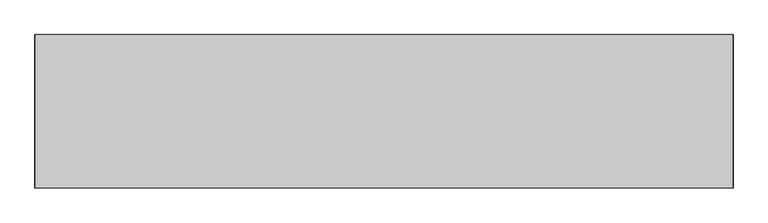
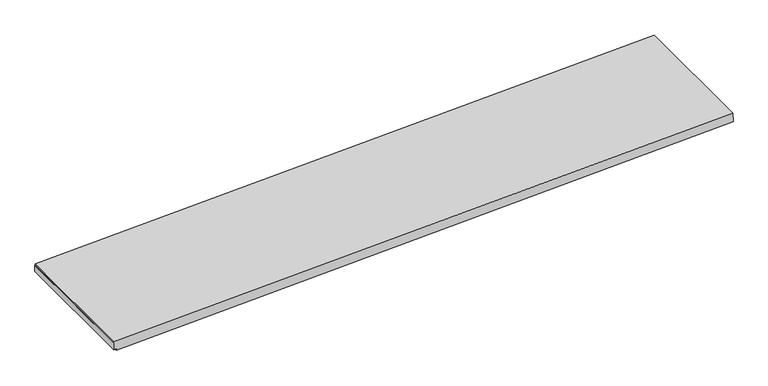
"""IFC4 building model written with IfcOpenShell, lengths in millimetres: proxy geometry, Generic Models 7:Generic Models 1:337419:Generic Models 1:337419 : Generic Models 7:Generic Models 1:337419:37 : Generic Models 7:Generic Models 1:337419:Generic Models 1:337419 : Generic Models 7:Generic Models 1:337419:301336."""

from ifc_helpers import new_model, si_unit, frame, origin, place, context, project, spatial, polyline, outline, extrude, source, transform, mapped, element, save


def generic_models_d0dfc169(model_context):
    return source(origin(), model_context, "Body", "SweptSolid", [
        extrude(outline(polyline([(4443.2315574, 579072.7180928), (4728.8631453, 579060.8167767), (3947.5164135, 560308.4952127), (3909.4494434, 560310.0813364), (3908.921022, 560297.3992239), (3708.5313384, 560297.3992239), (3708.5313384, 560373.112838), (3664.0813384, 560373.112838), (4443.2315574, 579072.7180928)])), frame((0.0, -578778.4413841, 0.0), z_axis=(0.0, 1.0, 0.0), x_axis=(0.0, 0.0, 1.0)), (0.0, 0.0, 1.0), 4126.5124605),
    ])


if __name__ == "__main__":
    model = new_model("IFC4")
    model_context = context("Model", 3, world=origin())
    ifc_project = project(units=[si_unit("LENGTHUNIT", "METRE", prefix="MILLI")], contexts=[model_context])
    site = spatial("IfcSite", under=ifc_project)
    building = spatial("IfcBuilding", under=site)
    placement = place(None, origin())
    generic_models_shape = generic_models_d0dfc169(model_context)
    element("IfcBuildingElementProxy", 1, Name="Generic Models 7:Generic Models 1:337419:Generic Models 1:337419 : Generic Models 7:Generic Models 1:337419:37 : Generic Models 7:Generic Models 1:337419:Generic Models 1:337419 : Generic Models 7:Generic Models 1:337419:301336", ObjectType="Generic Models 7:Generic Models 1:337419:Generic Models 1:337419 : Generic Models 7:Generic Models 1:337419:37 : Generic Models 7:Generic Models 1:337419:Generic Models 1:337419 : Generic Models 7:Generic Models 1:337419:301336", at=placement, inside=building, context=model_context, shape_type="MappedRepresentation", body=[
        mapped(generic_models_shape, transform((0.0, 0.0, 0.0), x_axis=(1.0, 0.0, 0.0), y_axis=(0.0, 1.0, 0.0), z_axis=(0.0, 0.0, 1.0))),
    ])
    save(model, "model.ifc")

# Revit data of these elements
# Type "Generic Models 7:Generic Models 1:337419:Generic Models 1:337419 : Generic Models 7:Generic Models 1:337419:37 : Generic Models 7:Generic Models 1:337419:Generic Models 1:337419 : Generic Models 7:Generic Models 1:337419:301336"
#   NameOverride = "Generic Models 7:Generic Models 1:337419:Generic Models 1:337419 : Generic Models 7:Generic Models 1:337419:301336"
#   ObjectTypeOverride = "Generic Models 1:337419 : Generic Models 7:Generic Models 1:337419"
#   Reference = "Generic Models 1"
#   Tag = "301336"
# Element 1 (IfcBuildingElementProxy, "Generic Models 7:Generic Models 1:337419:Generic Models 1:337419 : Generic Models 7:Generic Models 1:337419:37 : Generic Models 7:Generic Models 1:337419:Generic Models 1:337419 : Generic Models 7:Generic Models 1:337419:301336")
#   Materials on its faces: "SIMPLE SAVER INSULATION WITH LINER - COLOR: BLACK"
# Materials
#   "SIMPLE SAVER INSULATION WITH LINER - COLOR: BLACK": class "Unassigned", colour RGB 158 92 175, transparency 0, Cost = 0
